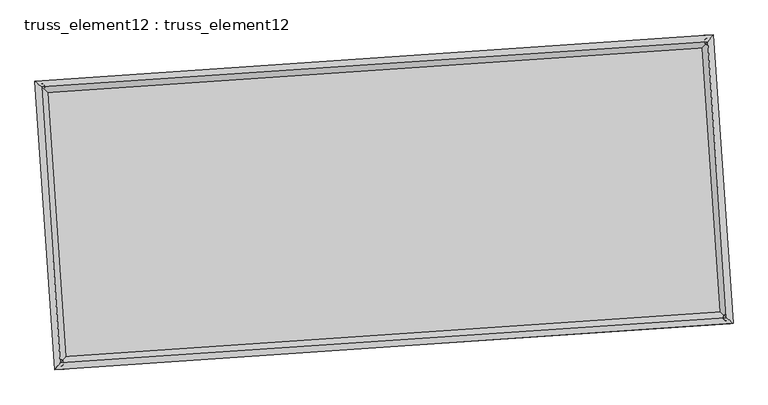
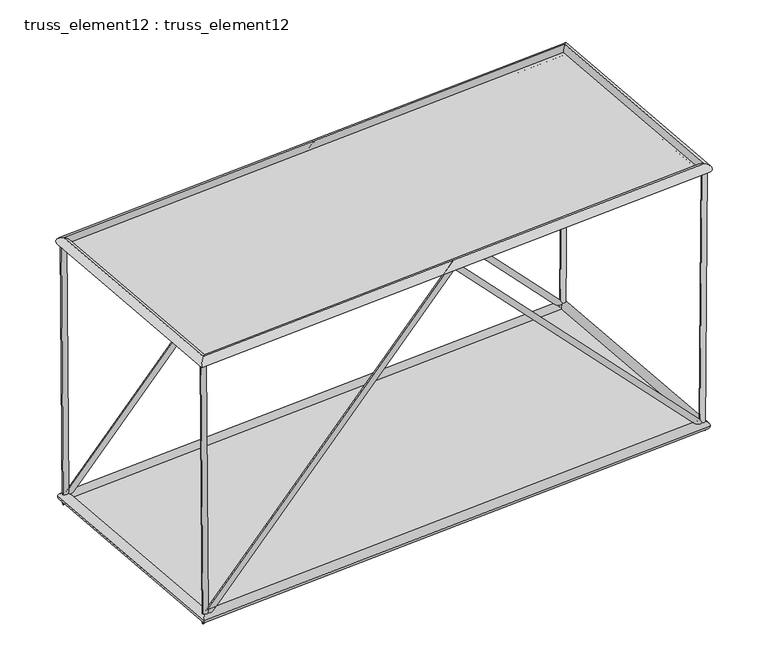
"""IFC4 building model written with IfcOpenShell, lengths in millimetres: plate geometry, truss_element12 : truss_element12."""

import ifcopenshell
import ifcopenshell.guid

model = None  # the IFC model being written
_history = None  # IfcOwnerHistory: only IFC2X3 demands one
_inside = {}  # id of a spatial element -> (the spatial element, [elements in it])
_under = {}  # id of a project, library or spatial element -> (it, [spatial elements below it])
_declared = {}  # id of a project -> (the project, [libraries it declares])
_typed = {}  # id of a type object -> (the type object, [elements of that type])
_made_of = {}  # id of a material, layer set ... -> (it, [elements and type objects made of it])


def new_model(schema):
    """Start an empty IFC model of exactly this schema.

    Asked for "IFC4X3", IfcOpenShell would pick the latest addendum, in which some entities
    have other attributes; the version numbers below select the first issue.
    IFC2X3 requires an IfcOwnerHistory on every rooted entity: one is made here for all.
    """
    global model, _history
    if schema == "IFC4X3":
        model = ifcopenshell.file(schema_version=(4, 3, 0, 0))
    else:
        model = ifcopenshell.file(schema=schema)
    _inside.clear()
    _under.clear()
    _declared.clear()
    _typed.clear()
    _made_of.clear()
    _history = None
    if model.schema == "IFC2X3":
        org = make("IfcOrganization", Name="unknown")
        user = make(
            "IfcPersonAndOrganization",
            ThePerson=make("IfcPerson", FamilyName="unknown"),
            TheOrganization=org,
        )
        app = make(
            "IfcApplication",
            ApplicationDeveloper=org,
            Version="unknown",
            ApplicationFullName="unknown",
            ApplicationIdentifier="unknown",
        )
        _history = make(
            "IfcOwnerHistory",
            OwningUser=user,
            OwningApplication=app,
            ChangeAction="ADDED",
            CreationDate=0,
        )
    return model


def make(cls, **values):
    """One entity of the class cls with the attributes given. An attribute that is None is left unset."""
    return model.create_entity(
        cls, **{name: value for name, value in values.items() if value is not None}
    )


def rooted(cls, **values):
    """An entity with a GlobalId (a new one), such as an element, a storey or a relation."""
    return make(cls, GlobalId=ifcopenshell.guid.new(), OwnerHistory=_history, **values)


def si_unit(unit_type, name, prefix=None):
    """IfcSIUnit, for example si_unit("LENGTHUNIT", "METRE", prefix="MILLI")."""
    return make("IfcSIUnit", UnitType=unit_type, Prefix=prefix, Name=name)


def assignment(units):
    """IfcUnitAssignment: the units of a project."""
    return None if units is None else make("IfcUnitAssignment", Units=units)


def point(xyz):
    """IfcCartesianPoint."""
    return None if xyz is None else make("IfcCartesianPoint", Coordinates=xyz)


def direction(xyz):
    """IfcDirection."""
    return None if xyz is None else make("IfcDirection", DirectionRatios=xyz)


def frame(location, z_axis=None, x_axis=None):
    """IfcAxis2Placement3D, a coordinate frame: its origin and axes. An axis left out is left unset."""
    return make(
        "IfcAxis2Placement3D",
        Location=point(location),
        Axis=direction(z_axis),
        RefDirection=direction(x_axis),
    )


def origin():
    """The frame at (0, 0, 0) with its axes left unset."""
    return frame((0.0, 0.0, 0.0))


def origin_with_axes():
    """The frame at (0, 0, 0) with the z axis (0, 0, 1) and the x axis (1, 0, 0) written out."""
    return frame((0.0, 0.0, 0.0), z_axis=(0.0, 0.0, 1.0), x_axis=(1.0, 0.0, 0.0))


def place(relative_to, where):
    """IfcLocalPlacement: puts the frame where relative to a parent placement (None: the world)."""
    return make(
        "IfcLocalPlacement", PlacementRelTo=relative_to, RelativePlacement=where
    )


def context(
    kind, dimensions, precision=None, world=None, true_north=None, identifier=None
):
    """IfcGeometricRepresentationContext, for example the 3D "Model" context."""
    return make(
        "IfcGeometricRepresentationContext",
        ContextIdentifier=identifier,
        ContextType=kind,
        CoordinateSpaceDimension=dimensions,
        Precision=precision,
        WorldCoordinateSystem=world,
        TrueNorth=true_north,
    )


def project(units=None, contexts=None):
    """IfcProject with its units and contexts."""
    return rooted(
        "IfcProject",
        Name="project",
        RepresentationContexts=contexts,
        UnitsInContext=assignment(units),
    )


def spatial(cls, under=None, at=None, **own):
    """A site, building, storey or space (cls), placed at a placement, below another one or the project."""
    s = rooted(cls, ObjectPlacement=at, **own)
    if under is not None:
        _under.setdefault(under.id(), (under, []))[1].append(s)
    return s


def polyline(points):
    """IfcPolyline through the points."""
    return make("IfcPolyline", Points=[point(p) for p in points])


def circle_curve(where, radius):
    """IfcCircle in the frame where."""
    return make("IfcCircle", Position=where, Radius=radius)


def ellipse_curve(where, semi_axis1, semi_axis2):
    """IfcEllipse in the frame where."""
    return make(
        "IfcEllipse", Position=where, SemiAxis1=semi_axis1, SemiAxis2=semi_axis2
    )


def outline(outer, holes=None, kind="AREA"):
    """IfcArbitraryClosedProfileDef: a profile drawn as a closed curve; with holes, ...WithVoids."""
    if holes is None:
        return make("IfcArbitraryClosedProfileDef", ProfileType=kind, OuterCurve=outer)
    return make(
        "IfcArbitraryProfileDefWithVoids",
        ProfileType=kind,
        OuterCurve=outer,
        InnerCurves=holes,
    )


def extrude(swept, where, along, depth):
    """IfcExtrudedAreaSolid: the profile swept, set in the frame where, extruded along a direction by depth."""
    return make(
        "IfcExtrudedAreaSolid",
        SweptArea=swept,
        Position=where,
        ExtrudedDirection=direction(along),
        Depth=depth,
    )


def shape(context_of_items, identifier, shape_type, items):
    """IfcShapeRepresentation: the items that make up one representation, for example the "Body"."""
    return make(
        "IfcShapeRepresentation",
        ContextOfItems=context_of_items,
        RepresentationIdentifier=identifier,
        RepresentationType=shape_type,
        Items=items,
    )


def source(mapping_origin, context_of_items, identifier, shape_type, items):
    """IfcRepresentationMap: a shape defined once, which mapped items show again and again."""
    return make(
        "IfcRepresentationMap",
        MappingOrigin=mapping_origin,
        MappedRepresentation=shape(context_of_items, identifier, shape_type, items),
    )


def transform(
    local_origin,
    x_axis=None,
    y_axis=None,
    z_axis=None,
    scale=None,
    scale2=None,
    scale3=None,
    uniform=True,
):
    """IfcCartesianTransformationOperator3D, or its non-uniform kind. x_axis, y_axis, z_axis: its Axis1, 2, 3."""
    if uniform:
        return make(
            "IfcCartesianTransformationOperator3D",
            Axis1=direction(x_axis),
            Axis2=direction(y_axis),
            LocalOrigin=point(local_origin),
            Scale=scale,
            Axis3=direction(z_axis),
        )
    return make(
        "IfcCartesianTransformationOperator3DnonUniform",
        Axis1=direction(x_axis),
        Axis2=direction(y_axis),
        LocalOrigin=point(local_origin),
        Scale=scale,
        Axis3=direction(z_axis),
        Scale2=scale2,
        Scale3=scale3,
    )


def mapped(mapping_source, mapping_target):
    """IfcMappedItem: shows the shape of a source again, moved by a transform."""
    return make(
        "IfcMappedItem", MappingSource=mapping_source, MappingTarget=mapping_target
    )


def made_of(thing, what):
    """Note that an element or type object is made of a material, layer set ...; save() writes the relation."""
    if what is not None:
        _made_of.setdefault(what.id(), (what, []))[1].append(thing)
    return thing


def element(
    cls,
    number,
    at=None,
    inside=None,
    cuts=None,
    type_object=None,
    material=None,
    context=None,
    identifier="Body",
    shape_type=None,
    held_by="IfcProductDefinitionShape",
    body=None,
    shapes=None,
    **own,
):
    """One element of the class cls, such as IfcWall. Its Tag is "e" and its number.

    at: its placement. inside: the storey or other place that contains it. cuts: it is an
    opening in that element (IfcRelVoidsElement). A single representation is given by context,
    identifier, shape_type and body (its items); several are given by shapes. held_by: the class
    of the entity that holds the representations. save() writes the other relations.
    """
    e = rooted(cls, Tag="e%d" % number, ObjectPlacement=at, **own)
    if body is not None:
        shapes = [shape(context, identifier, shape_type, body)]
    if shapes is not None:
        e.Representation = make(held_by, Representations=shapes)
    if inside is not None:
        _inside.setdefault(inside.id(), (inside, []))[1].append(e)
    if cuts is not None:
        rooted(
            "IfcRelVoidsElement", RelatingBuildingElement=cuts, RelatedOpeningElement=e
        )
    if type_object is not None:
        _typed.setdefault(type_object.id(), (type_object, []))[1].append(e)
    return made_of(e, material)


def aggregate(whole, parts):
    """IfcRelAggregates: a whole, such as a stair, and the parts it consists of."""
    return rooted("IfcRelAggregates", RelatingObject=whole, RelatedObjects=parts)


def save(model, path):
    """Write the relations noted so far, then the file.

    IfcRelAggregates (storeys below a building ...), IfcRelContainedInSpatialStructure (elements
    in a storey), IfcRelDefinesByType, IfcRelAssociatesMaterial and IfcRelDeclares: one each for
    every whole, place, type object, material and project.
    """
    for whole, parts in _under.values():
        aggregate(whole, parts)
    for where, things in _inside.values():
        rooted(
            "IfcRelContainedInSpatialStructure",
            RelatedElements=things,
            RelatingStructure=where,
        )
    for kind, things in _typed.values():
        rooted("IfcRelDefinesByType", RelatedObjects=things, RelatingType=kind)
    for what, things in _made_of.values():
        rooted("IfcRelAssociatesMaterial", RelatedObjects=things, RelatingMaterial=what)
    for by, libraries in _declared.values():
        rooted("IfcRelDeclares", RelatingContext=by, RelatedDefinitions=libraries)
    model.write(path)


def plane_surface(at):
    """IfcPlane: the flat surface through the origin of the frame at, square to its z axis."""
    return make("IfcPlane", Position=at)


def cylinder_surface(at, radius):
    """IfcCylindricalSurface: all points at the distance radius from the z axis of the frame at."""
    return make("IfcCylindricalSurface", Position=at, Radius=radius)


def advanced_brep(points, edges, surfaces, faces):
    """IfcAdvancedBrep: a solid bounded by faces that lie on surfaces and meet in shared edges.

    An edge is (start, end): straight between two places in points (the first is 0);
    or (start, end, curve); or (start, end, curve, False) where it runs against its curve.
    A face is (place in surfaces, loops), or (place, loops, False) where it looks against
    its surface's normal. A loop lists edges by number (the first is 1), with a minus sign
    where the edge is run from its end to its start. The first loop is the outer one.
    """
    corners = [point(p) for p in points]
    vertices = [make("IfcVertexPoint", VertexGeometry=c) for c in corners]
    made = []
    for start, end, *more in edges:
        made.append(
            make(
                "IfcEdgeCurve",
                EdgeStart=vertices[start],
                EdgeEnd=vertices[end],
                EdgeGeometry=more[0] if more else make("IfcPolyline", Points=[corners[start], corners[end]]),
                SameSense=more[1] if len(more) > 1 else True,
            )
        )
    hull = []
    for where, loops, *sense in faces:
        bounds = []
        for j, loop in enumerate(loops):
            ring = [make("IfcOrientedEdge", EdgeElement=made[abs(k) - 1], Orientation=k > 0) for k in loop]
            bounds.append(
                make(
                    "IfcFaceOuterBound" if j == 0 else "IfcFaceBound",
                    Bound=make("IfcEdgeLoop", EdgeList=ring),
                    Orientation=True,
                )
            )
        hull.append(make("IfcAdvancedFace", Bounds=bounds, FaceSurface=surfaces[where], SameSense=sense[0] if sense else True))
    return make("IfcAdvancedBrep", Outer=make("IfcClosedShell", CfsFaces=hull))


def truss_element12_truss_element12_eab3e817(model_context):
    return source(origin(), model_context, "Body", "SolidModel", [
        advanced_brep(
        [(-3702.0882248, 2273.6910917, 5000.2328853), (-3801.1888293, 2260.330024, 4999.4898764), (-3665.8559791, 2276.1616308, 123.2430264), (-3763.1309037, 2262.9250493, -123.2430264), (1064.0216291, 2598.674005, 5071.9820203), (1064.4653189, 2592.1004843, 4927.7362277), (5793.3095347, 2921.1461695, 123.2387731), (5891.4514423, 2921.234319, -123.2387731), (5830.1270154, 2923.6566136, 5000.2343714), (5930.1239348, 2923.8712492, 4999.4793629)],
        [
            (0, 1, circle_curve(frame((-3751.638527, 2267.0105579, 4999.8613808), z_axis=(-0.00742901712052106, -0.0005065564371103783, 0.9999722761682941), x_axis=(-0.13361073627191278, 0.991033768581535, -0.0004905955135681844)), 50.0)),
            (1, 0, circle_curve(frame((-3751.638527, 2267.0105579, 4999.8613808), z_axis=(-0.00742901712052106, -0.0005065564371103783, 0.9999722761682941), x_axis=(-0.13361073627191278, 0.991033768581535, -0.0004905955135681844)), 50.0)),
            (0, 2),
            (2, 3, ellipse_curve(frame((-3714.4934414, 2269.54334, 0.0), z_axis=(-0.9271592320010837, -0.06321946356795351, 0.36929535326258994), x_axis=(0.3684398421976921, 0.025122512268499236, 0.9293120800133068)), 132.9062538, 50.0)),
            (3, 1),
            (3, 2, ellipse_curve(frame((-3714.4934414, 2269.54334, 0.0), z_axis=(-0.9271592320010837, -0.06321946356795351, 0.36929535326258994), x_axis=(0.3684398421976921, 0.025122512268499236, 0.9293120800133068)), 132.9062538, 50.0)),
            (2, 4),
            (4, 5, ellipse_curve(frame((1064.243474, 2595.3872446, 4999.859124), z_axis=(-0.9976833955843889, -0.0680282381952549, 3.1356873965195084e-05), x_axis=(-3.128423250774107e-05, -2.1331528923241756e-06, -0.9999999995083731)), 72.2799434, 50.0)),
            (5, 3),
            (5, 4, ellipse_curve(frame((1064.243474, 2595.3872446, 4999.859124), z_axis=(-0.9976833955843889, -0.0680282381952549, 3.1356873965195084e-05), x_axis=(-3.128423250774107e-05, -2.1331528923241756e-06, -0.9999999995083731)), 72.2799434, 50.0)),
            (4, 6),
            (6, 7, ellipse_curve(frame((5842.3804885, 2921.1902443, 0.0), z_axis=(-0.9271929359308114, -0.06322176171080063, -0.369210330849754), x_axis=(-0.3683550167481115, -0.025116728343544018, 0.929345862202988)), 132.8968359, 50.0)),
            (7, 5),
            (7, 6, ellipse_curve(frame((5842.3804885, 2921.1902443, 0.0), z_axis=(-0.9271929359308114, -0.06322176171080063, -0.369210330849754), x_axis=(-0.3683550167481115, -0.025116728343544018, 0.929345862202988)), 132.8968359, 50.0)),
            (8, 9, circle_curve(frame((5880.1254751, 2923.7639314, 4999.8568672), z_axis=(0.007548997314579444, 0.0005147374304556931, 0.999971373432721), x_axis=(-0.002150181299370391, 0.9999975640967588, -0.0004985187346304086)), 50.0)),
            (9, 8, circle_curve(frame((5880.1254751, 2923.7639314, 4999.8568672), z_axis=(0.007548997314579444, 0.0005147374304556931, 0.999971373432721), x_axis=(-0.002150181299370391, 0.9999975640967588, -0.0004985187346304086)), 50.0)),
            (6, 8),
            (9, 7),
        ],
        [
            plane_surface(frame((-3751.638527, 2317.0105514, 4999.8867094), z_axis=(-0.007429017120522367, -0.0005065564371127931, 0.9999722761682941), x_axis=(0.9999724044715549, -3.7633202945031043e-06, 0.007429016167328942))),
            cylinder_surface(frame((-3751.638527, 2267.0105579, 4999.8613808), z_axis=(-0.00742901712052106, -0.0005065564371103783, 0.9999722761682941), x_axis=(-0.13361073627191278, 0.991033768581535, -0.0004905955135681844)), 50.0),
            cylinder_surface(frame((-3714.4934414, 2269.54334, 0.0), z_axis=(-0.6901748995971244, -0.04706040280311354, -0.7221107438988209), x_axis=(-0.020414552183437053, 0.998752186075548, -0.045577591736113365)), 50.0),
            cylinder_surface(frame((1064.243474, 2595.3872446, 4999.859124), z_axis=(-0.6901297168790954, -0.047057321965326554, 0.7221541264368925), x_axis=(-0.11534915767572501, 0.9922789562072498, -0.04557460797145166)), 50.0),
            plane_surface(frame((5880.1254751, 2873.763938, 4999.8826048), z_axis=(0.007548997314579199, 0.0005147374304560268, 0.999971373432721), x_axis=(0.9999715059138159, -3.885862204455747e-06, -0.007548996314451271))),
            cylinder_surface(frame((5842.3804885, 2921.1902443, 0.0), z_axis=(-0.007548997314579444, -0.0005147374304556931, -0.999971373432721), x_axis=(-0.002150181299370391, 0.9999975640967588, -0.0004985187346304086)), 50.0),
        ],
        [
            (0, [[1, 2]]),
            (1, [[-1, 3, 4, 5]]),
            (1, [[-2, -5, 6, -3]]),
            (2, [[-4, 7, 8, 9]]),
            (2, [[-6, -9, 10, -7]]),
            (3, [[-8, 11, 12, 13]]),
            (3, [[-10, -13, 14, -11]]),
            (4, [[15, 16]]),
            (5, [[-12, 17, -16, 18]]),
            (5, [[-14, -18, -15, -17]]),
        ],
    ),
        advanced_brep(
        [(-3429.9752719, -1717.0424926, 5000.2328853), (-3529.0758763, -1730.4035603, 4999.4898764), (-3393.7430262, -1714.5719535, 123.2430264), (-3491.0179508, -1727.808535, -123.2430264), (1336.1345821, -1392.0595793, 5071.9820203), (1336.5782718, -1398.6331, 4927.7362277), (6065.4224876, -1069.5874148, 123.2387731), (6163.5643952, -1069.4992653, -123.2387731), (6102.2399683, -1067.0769707, 5000.2343714), (6202.2368877, -1066.8623351, 4999.4793629)],
        [
            (0, 1, circle_curve(frame((-3479.5255741, -1723.7230264, 4999.8613808), z_axis=(-0.007429017120521156, -0.0005065564371104173, 0.9999722761682941), x_axis=(-0.1336107362719125, 0.9910337685815351, -0.0004905955135681566)), 50.0)),
            (1, 0, circle_curve(frame((-3479.5255741, -1723.7230264, 4999.8613808), z_axis=(-0.007429017120521156, -0.0005065564371104173, 0.9999722761682941), x_axis=(-0.1336107362719125, 0.9910337685815351, -0.0004905955135681566)), 50.0)),
            (0, 2),
            (2, 3, ellipse_curve(frame((-3442.3804885, -1721.1902443, 0.0), z_axis=(-0.9271592320010837, -0.06321946356795342, 0.3692953532625894), x_axis=(0.3684398421976915, 0.025122512268499122, 0.929312080013307)), 132.9062538, 50.0)),
            (3, 1),
            (3, 2, ellipse_curve(frame((-3442.3804885, -1721.1902443, 0.0), z_axis=(-0.9271592320010837, -0.06321946356795342, 0.3692953532625894), x_axis=(0.3684398421976915, 0.025122512268499122, 0.929312080013307)), 132.9062538, 50.0)),
            (2, 4),
            (4, 5, ellipse_curve(frame((1336.3564269, -1395.3463397, 4999.859124), z_axis=(-0.9976833955843889, -0.068028238195255, 3.135687396423212e-05), x_axis=(-3.128423250681861e-05, -2.1331528920455174e-06, -0.9999999995083731)), 72.2799434, 50.0)),
            (5, 3),
            (5, 4, ellipse_curve(frame((1336.3564269, -1395.3463397, 4999.859124), z_axis=(-0.9976833955843889, -0.068028238195255, 3.135687396423212e-05), x_axis=(-3.128423250681861e-05, -2.1331528920455174e-06, -0.9999999995083731)), 72.2799434, 50.0)),
            (4, 6),
            (6, 7, ellipse_curve(frame((6114.4934414, -1069.54334, 0.0), z_axis=(-0.9271929359308113, -0.06322176171080102, -0.36921033084975446), x_axis=(-0.36835501674811183, -0.025116728343544108, 0.9293458622029878)), 132.8968359, 50.0)),
            (7, 5),
            (7, 6, ellipse_curve(frame((6114.4934414, -1069.54334, 0.0), z_axis=(-0.9271929359308113, -0.06322176171080102, -0.36921033084975446), x_axis=(-0.36835501674811183, -0.025116728343544108, 0.9293458622029878)), 132.8968359, 50.0)),
            (8, 9, circle_curve(frame((6152.238428, -1066.9696529, 4999.8568672), z_axis=(0.0075489973145789376, 0.0005147374304557482, 0.9999713734327209), x_axis=(-0.002150181299370522, 0.9999975640967588, -0.0004985187346304639)), 50.0)),
            (9, 8, circle_curve(frame((6152.238428, -1066.9696529, 4999.8568672), z_axis=(0.0075489973145789376, 0.0005147374304557482, 0.9999713734327209), x_axis=(-0.002150181299370522, 0.9999975640967588, -0.0004985187346304639)), 50.0)),
            (6, 8),
            (9, 7),
        ],
        [
            plane_surface(frame((-3479.5255741, -1673.7230329, 4999.8867094), z_axis=(-0.007429017120522367, -0.000506556437112789, 0.9999722761682941), x_axis=(0.9999724044715549, -3.7633202945031043e-06, 0.007429016167328942))),
            cylinder_surface(frame((-3479.5255741, -1723.7230264, 4999.8613808), z_axis=(-0.007429017120521158, -0.0005065564371104174, 0.9999722761682943), x_axis=(-0.1336107362719125, 0.9910337685815351, -0.0004905955135681566)), 50.0),
            cylinder_surface(frame((-3442.3804885, -1721.1902443, 0.0), z_axis=(-0.6901748995971234, -0.04706040280311338, -0.7221107438988217), x_axis=(-0.020414552183436876, 0.998752186075548, -0.0455775917361133)), 50.0),
            cylinder_surface(frame((1336.3564269, -1395.3463397, 4999.859124), z_axis=(-0.6901297168790961, -0.04705732196532681, 0.7221541264368919), x_axis=(-0.11534915767572519, 0.9922789562072498, -0.04557460797145163)), 50.0),
            plane_surface(frame((6152.238428, -1116.9696463, 4999.8826048), z_axis=(0.007548997314579199, 0.0005147374304560219, 0.999971373432721), x_axis=(0.9999715059138159, -3.885862204455747e-06, -0.007548996314451271))),
            cylinder_surface(frame((6114.4934414, -1069.54334, 0.0), z_axis=(-0.007548997314578939, -0.0005147374304557483, -0.9999713734327211), x_axis=(-0.002150181299370522, 0.9999975640967588, -0.0004985187346304639)), 50.0),
        ],
        [
            (0, [[1, 2]]),
            (1, [[-1, 3, 4, 5]]),
            (1, [[-2, -5, 6, -3]]),
            (2, [[-4, 7, 8, 9]]),
            (2, [[-6, -9, 10, -7]]),
            (3, [[-8, 11, 12, 13]]),
            (3, [[-10, -13, 14, -11]]),
            (4, [[15, 16]]),
            (5, [[-12, 17, -16, 18]]),
            (5, [[-14, -18, -15, -17]]),
        ],
    ),
        advanced_brep(
        [(-3479.5267648, -1723.7243462, 4909.8613809), (-3479.5243834, -1723.7217067, 5089.8613808), (-3751.6371682, 2267.009412, 5089.8613808), (-3751.6398859, 2267.0117037, 4909.8613809), (5880.1243683, 2923.7626174, 5089.8568672), (5880.1265818, 2923.7652454, 4909.8568672), (6152.2371531, -1066.9685013, 5089.8568672), (6152.2397029, -1066.9708045, 4909.8568672)],
        [
            (0, 1, ellipse_curve(frame((-3479.5255741, -1723.7230264, 4999.8613808), z_axis=(-0.7535719234053809, 0.6573654662780861, 3.30599714592259e-07), x_axis=(-0.6573654662780039, -0.7535719234054525, 3.305997145922409e-07)), 127.2792206, 90.0)),
            (1, 2),
            (2, 3, ellipse_curve(frame((-3751.638527, 2267.0105579, 4999.8613808), z_axis=(-0.6573654662780037, -0.7535719234054528, 3.3059971459222477e-07), x_axis=(0.7535719234053809, -0.657365466278086, -3.305997145922429e-07)), 127.2792206, 90.0)),
            (3, 0),
            (1, 0, ellipse_curve(frame((-3479.5255741, -1723.7230264, 4999.8613808), z_axis=(-0.7535719234053809, 0.6573654662780861, 3.30599714592259e-07), x_axis=(-0.6573654662780039, -0.7535719234054525, 3.305997145922409e-07)), 127.2792206, 90.0)),
            (3, 2, ellipse_curve(frame((-3751.638527, 2267.0105579, 4999.8613808), z_axis=(-0.6573654662780037, -0.7535719234054528, 3.3059971459222477e-07), x_axis=(0.7535719234053809, -0.657365466278086, -3.305997145922429e-07)), 127.2792206, 90.0)),
            (2, 4),
            (4, 5, ellipse_curve(frame((5880.1254751, 2923.7639314, 4999.8568672), z_axis=(-0.7535719234053808, 0.6573654662780862, 3.3059971459222667e-07), x_axis=(-0.6573654662780037, -0.7535719234054528, 3.3059971459224097e-07)), 127.2792206, 90.0)),
            (5, 3),
            (5, 4, ellipse_curve(frame((5880.1254751, 2923.7639314, 4999.8568672), z_axis=(-0.7535719234053808, 0.6573654662780862, 3.3059971459222667e-07), x_axis=(-0.6573654662780037, -0.7535719234054528, 3.3059971459224097e-07)), 127.2792206, 90.0)),
            (4, 6),
            (6, 7, ellipse_curve(frame((6152.238428, -1066.9696529, 4999.8568672), z_axis=(0.6573654662780037, 0.7535719234054526, -3.3059971459225706e-07), x_axis=(-0.7535719234053807, 0.6573654662780862, 3.3059971459224277e-07)), 127.2792206, 90.0)),
            (7, 5),
            (7, 6, ellipse_curve(frame((6152.238428, -1066.9696529, 4999.8568672), z_axis=(0.6573654662780037, 0.7535719234054526, -3.3059971459225706e-07), x_axis=(-0.7535719234053807, 0.6573654662780862, 3.3059971459224277e-07)), 127.2792206, 90.0)),
            (6, 1),
            (0, 7),
        ],
        [
            cylinder_surface(frame((-3479.5255741, -1723.7230264, 4999.8613808), z_axis=(0.06802823822870098, -0.9976833960748767, 0.0), x_axis=(-0.9976833959743321, -0.06802823822184523, 1.4197044503846432e-05)), 90.0),
            cylinder_surface(frame((-3751.638527, 2267.0105579, 4999.8613808), z_axis=(-0.9976833960747676, -0.06802823822869408, 4.6753860009301154e-07), x_axis=(-0.06802823821588568, 0.997683395981282, 1.3729505903797475e-05)), 90.0),
            cylinder_surface(frame((5880.1254751, 2923.7639314, 4999.8568672), z_axis=(-0.06802823822870059, 0.9976833960748767, 0.0), x_axis=(0.9976833959871405, 0.0680282382227182, 1.3261967303748516e-05)), 90.0),
            cylinder_surface(frame((6152.238428, -1066.9696529, 4999.8568672), z_axis=(0.9976833960747675, 0.06802823822869422, -4.6753860009303425e-07), x_axis=(0.06802823822869422, -0.9976833959804086, 1.3729505903797473e-05)), 90.0),
        ],
        [
            (0, [[1, 2, 3, 4]]),
            (0, [[5, -4, 6, -2]]),
            (1, [[-3, 7, 8, 9]]),
            (1, [[-6, -9, 10, -7]]),
            (2, [[-8, 11, 12, 13]]),
            (2, [[-10, -13, 14, -11]]),
            (3, [[-12, 15, -1, 16]]),
            (3, [[-14, -16, -5, -15]]),
        ],
    ),
        advanced_brep(
        [(-3358.7115243, -1625.2761972, 0.0), (-3526.0494527, -1817.1042913, 0.0), (-3810.4074885, 2353.2123043, 0.0), (-3618.5793943, 2185.8743758, 0.0), (5926.0494527, 3017.1042913, 0.0), (5758.7115243, 2825.2761972, 0.0), (6210.4074885, -1153.2123043, 0.0), (6018.5793943, -985.8743758, 0.0)],
        [
            (0, 1, ellipse_curve(frame((-3442.3804885, -1721.1902443, 0.0), z_axis=(-0.7535719234054562, 0.6573654662780827, 0.0), x_axis=(-0.6573654662780827, -0.7535719234054564, 0.0)), 127.2792206, 90.0)),
            (1, 2),
            (2, 3, ellipse_curve(frame((-3714.4934414, 2269.54334, 0.0), z_axis=(-0.6573654662780826, -0.7535719234054563, 0.0), x_axis=(0.7535719234054563, -0.6573654662780828, 0.0)), 127.2792206, 90.0)),
            (3, 0),
            (1, 0, ellipse_curve(frame((-3442.3804885, -1721.1902443, 0.0), z_axis=(-0.7535719234054562, 0.6573654662780827, 0.0), x_axis=(-0.6573654662780827, -0.7535719234054564, 0.0)), 127.2792206, 90.0)),
            (3, 2, ellipse_curve(frame((-3714.4934414, 2269.54334, 0.0), z_axis=(-0.6573654662780826, -0.7535719234054563, 0.0), x_axis=(0.7535719234054563, -0.6573654662780828, 0.0)), 127.2792206, 90.0)),
            (2, 4),
            (4, 5, ellipse_curve(frame((5842.3804885, 2921.1902443, 0.0), z_axis=(-0.7535719234054563, 0.6573654662780827, 0.0), x_axis=(-0.6573654662780828, -0.7535719234054563, 0.0)), 127.2792206, 90.0)),
            (5, 3),
            (5, 4, ellipse_curve(frame((5842.3804885, 2921.1902443, 0.0), z_axis=(-0.7535719234054563, 0.6573654662780827, 0.0), x_axis=(-0.6573654662780828, -0.7535719234054563, 0.0)), 127.2792206, 90.0)),
            (4, 6),
            (6, 7, ellipse_curve(frame((6114.4934414, -1069.54334, 0.0), z_axis=(0.6573654662780828, 0.7535719234054562, 0.0), x_axis=(-0.7535719234054563, 0.6573654662780828, 0.0)), 127.2792206, 90.0)),
            (7, 5),
            (7, 6, ellipse_curve(frame((6114.4934414, -1069.54334, 0.0), z_axis=(0.6573654662780828, 0.7535719234054562, 0.0), x_axis=(-0.7535719234054563, 0.6573654662780828, 0.0)), 127.2792206, 90.0)),
            (6, 1),
            (0, 7),
        ],
        [
            cylinder_surface(frame((-3442.3804885, -1721.1902443, 0.0), z_axis=(0.06802823822869855, -0.9976833960748768, 0.0), x_axis=(-0.9976833960748768, -0.06802823822869855, 0.0)), 90.0),
            cylinder_surface(frame((-3714.4934414, 2269.54334, 0.0), z_axis=(-0.9976833960748768, -0.0680282382286992, 0.0), x_axis=(-0.0680282382286992, 0.9976833960748768, 0.0)), 90.0),
            cylinder_surface(frame((5842.3804885, 2921.1902443, 0.0), z_axis=(-0.0680282382286982, 0.9976833960748769, 0.0), x_axis=(0.9976833960748769, 0.0680282382286982, 0.0)), 90.0),
            cylinder_surface(frame((6114.4934414, -1069.54334, 0.0), z_axis=(0.9976833960748768, 0.06802823822869884, 0.0), x_axis=(0.06802823822869884, -0.9976833960748768, 0.0)), 90.0),
        ],
        [
            (0, [[1, 2, 3, 4]]),
            (0, [[5, -4, 6, -2]]),
            (1, [[-3, 7, 8, 9]]),
            (1, [[-6, -9, 10, -7]]),
            (2, [[-8, 11, 12, 13]]),
            (2, [[-10, -13, 14, -11]]),
            (3, [[-12, 15, -1, 16]]),
            (3, [[-14, -16, -5, -15]]),
        ],
    ),
        extrude(outline(polyline([(-3442.3804885, -1721.1902443), (-3714.4934414, 2269.54334), (5842.3804885, 2921.1902443), (6114.4934414, -1069.54334), (-3442.3804885, -1721.1902443)])), origin_with_axes(), (0.0, 0.0, 1.0), 20.0),
        extrude(outline(polyline([(-2000.0, 4827.0643974), (2000.0, 4827.0643974), (2000.0, -4827.0643974), (-2000.0, -4827.0643974), (-2000.0, 4827.0643974)])), frame((1200.2999505, 600.0204525, 4999.859124), z_axis=(4.664554983369009e-07, 3.180582726824052e-08, 0.9999999999998908), x_axis=(-0.06802823822869884, 0.9976833960748768, 0.0)), (0.0, 0.0, 1.0), 20.0),
    ])


if __name__ == "__main__":
    model = new_model("IFC4")
    model_context = context("Model", 3, world=origin())
    ifc_project = project(units=[si_unit("LENGTHUNIT", "METRE", prefix="MILLI")], contexts=[model_context])
    site = spatial("IfcSite", under=ifc_project)
    building = spatial("IfcBuilding", under=site)
    placement = place(None, origin())
    truss_element12_truss_element12_shape = truss_element12_truss_element12_eab3e817(model_context)
    element("IfcPlate", 1, ObjectType="truss_element12 : truss_element12", at=placement, inside=building, context=model_context, shape_type="MappedRepresentation", body=[
        mapped(truss_element12_truss_element12_shape, transform((0.0, 0.0, 0.0), x_axis=(1.0, 0.0, 0.0), y_axis=(0.0, 1.0, 0.0), z_axis=(0.0, 0.0, 1.0))),
    ])
    save(model, "model.ifc")

# Revit data of these elements
# Type "truss_element12 : truss_element12"
#   steellbar1 = 90 mm
#   steelbar2 = 50 mm
#   offset1 = 5000 mm
#   M = Default Roof
# Element 1 (IfcPlate, "truss_element12 : truss_element12")
#   Materials on its faces: "Default Roof"
# Materials
#   "Default Roof": class "Miscellaneous", colour RGB 0 127 0, transparency 0, Comments = "Rendering appearance not upgraded Rendering appearance not upgraded ", Cost = 0
